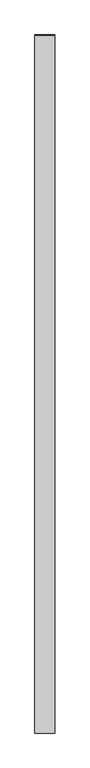
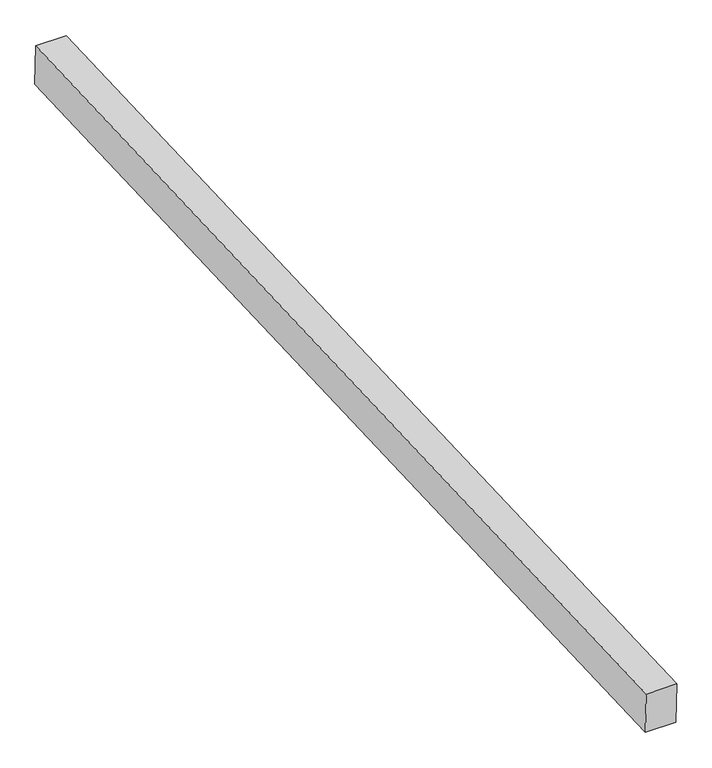
"""IFC4 building model written with IfcOpenShell, lengths in millimetres: proxy geometry, Generic Models 7:Generic Models 1:8:Generic Models 1:8 : Generic Models 7:Generic Models 1:337419:44 : Generic Models 7:Generic Models 1:8:Generic Models 1:8 : Generic Models 7:Generic Models 1:337419:315935."""

import ifcopenshell
import ifcopenshell.guid

model = None  # the IFC model being written
_history = None  # IfcOwnerHistory: only IFC2X3 demands one
_inside = {}  # id of a spatial element -> (the spatial element, [elements in it])
_under = {}  # id of a project, library or spatial element -> (it, [spatial elements below it])
_declared = {}  # id of a project -> (the project, [libraries it declares])
_typed = {}  # id of a type object -> (the type object, [elements of that type])
_made_of = {}  # id of a material, layer set ... -> (it, [elements and type objects made of it])


def new_model(schema):
    """Start an empty IFC model of exactly this schema.

    Asked for "IFC4X3", IfcOpenShell would pick the latest addendum, in which some entities
    have other attributes; the version numbers below select the first issue.
    IFC2X3 requires an IfcOwnerHistory on every rooted entity: one is made here for all.
    """
    global model, _history
    if schema == "IFC4X3":
        model = ifcopenshell.file(schema_version=(4, 3, 0, 0))
    else:
        model = ifcopenshell.file(schema=schema)
    _inside.clear()
    _under.clear()
    _declared.clear()
    _typed.clear()
    _made_of.clear()
    _history = None
    if model.schema == "IFC2X3":
        org = make("IfcOrganization", Name="unknown")
        user = make(
            "IfcPersonAndOrganization",
            ThePerson=make("IfcPerson", FamilyName="unknown"),
            TheOrganization=org,
        )
        app = make(
            "IfcApplication",
            ApplicationDeveloper=org,
            Version="unknown",
            ApplicationFullName="unknown",
            ApplicationIdentifier="unknown",
        )
        _history = make(
            "IfcOwnerHistory",
            OwningUser=user,
            OwningApplication=app,
            ChangeAction="ADDED",
            CreationDate=0,
        )
    return model


def make(cls, **values):
    """One entity of the class cls with the attributes given. An attribute that is None is left unset."""
    return model.create_entity(
        cls, **{name: value for name, value in values.items() if value is not None}
    )


def rooted(cls, **values):
    """An entity with a GlobalId (a new one), such as an element, a storey or a relation."""
    return make(cls, GlobalId=ifcopenshell.guid.new(), OwnerHistory=_history, **values)


def si_unit(unit_type, name, prefix=None):
    """IfcSIUnit, for example si_unit("LENGTHUNIT", "METRE", prefix="MILLI")."""
    return make("IfcSIUnit", UnitType=unit_type, Prefix=prefix, Name=name)


def assignment(units):
    """IfcUnitAssignment: the units of a project."""
    return None if units is None else make("IfcUnitAssignment", Units=units)


def point(xyz):
    """IfcCartesianPoint."""
    return None if xyz is None else make("IfcCartesianPoint", Coordinates=xyz)


def direction(xyz):
    """IfcDirection."""
    return None if xyz is None else make("IfcDirection", DirectionRatios=xyz)


def frame(location, z_axis=None, x_axis=None):
    """IfcAxis2Placement3D, a coordinate frame: its origin and axes. An axis left out is left unset."""
    return make(
        "IfcAxis2Placement3D",
        Location=point(location),
        Axis=direction(z_axis),
        RefDirection=direction(x_axis),
    )


def origin():
    """The frame at (0, 0, 0) with its axes left unset."""
    return frame((0.0, 0.0, 0.0))


def place(relative_to, where):
    """IfcLocalPlacement: puts the frame where relative to a parent placement (None: the world)."""
    return make(
        "IfcLocalPlacement", PlacementRelTo=relative_to, RelativePlacement=where
    )


def context(
    kind, dimensions, precision=None, world=None, true_north=None, identifier=None
):
    """IfcGeometricRepresentationContext, for example the 3D "Model" context."""
    return make(
        "IfcGeometricRepresentationContext",
        ContextIdentifier=identifier,
        ContextType=kind,
        CoordinateSpaceDimension=dimensions,
        Precision=precision,
        WorldCoordinateSystem=world,
        TrueNorth=true_north,
    )


def project(units=None, contexts=None):
    """IfcProject with its units and contexts."""
    return rooted(
        "IfcProject",
        Name="project",
        RepresentationContexts=contexts,
        UnitsInContext=assignment(units),
    )


def spatial(cls, under=None, at=None, **own):
    """A site, building, storey or space (cls), placed at a placement, below another one or the project."""
    s = rooted(cls, ObjectPlacement=at, **own)
    if under is not None:
        _under.setdefault(under.id(), (under, []))[1].append(s)
    return s


def polyline(points):
    """IfcPolyline through the points."""
    return make("IfcPolyline", Points=[point(p) for p in points])


def outline(outer, holes=None, kind="AREA"):
    """IfcArbitraryClosedProfileDef: a profile drawn as a closed curve; with holes, ...WithVoids."""
    if holes is None:
        return make("IfcArbitraryClosedProfileDef", ProfileType=kind, OuterCurve=outer)
    return make(
        "IfcArbitraryProfileDefWithVoids",
        ProfileType=kind,
        OuterCurve=outer,
        InnerCurves=holes,
    )


def extrude(swept, where, along, depth):
    """IfcExtrudedAreaSolid: the profile swept, set in the frame where, extruded along a direction by depth."""
    return make(
        "IfcExtrudedAreaSolid",
        SweptArea=swept,
        Position=where,
        ExtrudedDirection=direction(along),
        Depth=depth,
    )


def shape(context_of_items, identifier, shape_type, items):
    """IfcShapeRepresentation: the items that make up one representation, for example the "Body"."""
    return make(
        "IfcShapeRepresentation",
        ContextOfItems=context_of_items,
        RepresentationIdentifier=identifier,
        RepresentationType=shape_type,
        Items=items,
    )


def source(mapping_origin, context_of_items, identifier, shape_type, items):
    """IfcRepresentationMap: a shape defined once, which mapped items show again and again."""
    return make(
        "IfcRepresentationMap",
        MappingOrigin=mapping_origin,
        MappedRepresentation=shape(context_of_items, identifier, shape_type, items),
    )


def transform(
    local_origin,
    x_axis=None,
    y_axis=None,
    z_axis=None,
    scale=None,
    scale2=None,
    scale3=None,
    uniform=True,
):
    """IfcCartesianTransformationOperator3D, or its non-uniform kind. x_axis, y_axis, z_axis: its Axis1, 2, 3."""
    if uniform:
        return make(
            "IfcCartesianTransformationOperator3D",
            Axis1=direction(x_axis),
            Axis2=direction(y_axis),
            LocalOrigin=point(local_origin),
            Scale=scale,
            Axis3=direction(z_axis),
        )
    return make(
        "IfcCartesianTransformationOperator3DnonUniform",
        Axis1=direction(x_axis),
        Axis2=direction(y_axis),
        LocalOrigin=point(local_origin),
        Scale=scale,
        Axis3=direction(z_axis),
        Scale2=scale2,
        Scale3=scale3,
    )


def mapped(mapping_source, mapping_target):
    """IfcMappedItem: shows the shape of a source again, moved by a transform."""
    return make(
        "IfcMappedItem", MappingSource=mapping_source, MappingTarget=mapping_target
    )


def made_of(thing, what):
    """Note that an element or type object is made of a material, layer set ...; save() writes the relation."""
    if what is not None:
        _made_of.setdefault(what.id(), (what, []))[1].append(thing)
    return thing


def element(
    cls,
    number,
    at=None,
    inside=None,
    cuts=None,
    type_object=None,
    material=None,
    context=None,
    identifier="Body",
    shape_type=None,
    held_by="IfcProductDefinitionShape",
    body=None,
    shapes=None,
    **own,
):
    """One element of the class cls, such as IfcWall. Its Tag is "e" and its number.

    at: its placement. inside: the storey or other place that contains it. cuts: it is an
    opening in that element (IfcRelVoidsElement). A single representation is given by context,
    identifier, shape_type and body (its items); several are given by shapes. held_by: the class
    of the entity that holds the representations. save() writes the other relations.
    """
    e = rooted(cls, Tag="e%d" % number, ObjectPlacement=at, **own)
    if body is not None:
        shapes = [shape(context, identifier, shape_type, body)]
    if shapes is not None:
        e.Representation = make(held_by, Representations=shapes)
    if inside is not None:
        _inside.setdefault(inside.id(), (inside, []))[1].append(e)
    if cuts is not None:
        rooted(
            "IfcRelVoidsElement", RelatingBuildingElement=cuts, RelatedOpeningElement=e
        )
    if type_object is not None:
        _typed.setdefault(type_object.id(), (type_object, []))[1].append(e)
    return made_of(e, material)


def aggregate(whole, parts):
    """IfcRelAggregates: a whole, such as a stair, and the parts it consists of."""
    return rooted("IfcRelAggregates", RelatingObject=whole, RelatedObjects=parts)


def save(model, path):
    """Write the relations noted so far, then the file.

    IfcRelAggregates (storeys below a building ...), IfcRelContainedInSpatialStructure (elements
    in a storey), IfcRelDefinesByType, IfcRelAssociatesMaterial and IfcRelDeclares: one each for
    every whole, place, type object, material and project.
    """
    for whole, parts in _under.values():
        aggregate(whole, parts)
    for where, things in _inside.values():
        rooted(
            "IfcRelContainedInSpatialStructure",
            RelatedElements=things,
            RelatingStructure=where,
        )
    for kind, things in _typed.values():
        rooted("IfcRelDefinesByType", RelatedObjects=things, RelatingType=kind)
    for what, things in _made_of.values():
        rooted("IfcRelAssociatesMaterial", RelatedObjects=things, RelatingMaterial=what)
    for by, libraries in _declared.values():
        rooted("IfcRelDeclares", RelatingContext=by, RelatedDefinitions=libraries)
    model.write(path)


def generic_models_2becdbc0(model_context):
    return source(origin(), model_context, "Body", "SweptSolid", [
        extrude(outline(polyline([(-581229.2495411, 3818.908703), (-576356.3266468, 4021.9471569), (-576348.7597251, 3831.5971524), (-581221.3189223, 3628.5738526), (-581229.2495411, 3818.908703)])), frame((659844.7617239, 0.0, 0.0), z_axis=(1.0, 0.0, 0.0), x_axis=(0.0, 1.0, 0.0)), (0.0, 0.0, 1.0), 139.7),
    ])


if __name__ == "__main__":
    model = new_model("IFC4")
    model_context = context("Model", 3, world=origin())
    ifc_project = project(units=[si_unit("LENGTHUNIT", "METRE", prefix="MILLI")], contexts=[model_context])
    site = spatial("IfcSite", under=ifc_project)
    building = spatial("IfcBuilding", under=site)
    placement = place(None, origin())
    generic_models_shape = generic_models_2becdbc0(model_context)
    element("IfcBuildingElementProxy", 1, Name="Generic Models 7:Generic Models 1:8:Generic Models 1:8 : Generic Models 7:Generic Models 1:337419:44 : Generic Models 7:Generic Models 1:8:Generic Models 1:8 : Generic Models 7:Generic Models 1:337419:315935", ObjectType="Generic Models 7:Generic Models 1:8:Generic Models 1:8 : Generic Models 7:Generic Models 1:337419:44 : Generic Models 7:Generic Models 1:8:Generic Models 1:8 : Generic Models 7:Generic Models 1:337419:315935", at=placement, inside=building, context=model_context, shape_type="MappedRepresentation", body=[
        mapped(generic_models_shape, transform((0.0, 0.0, 0.0), x_axis=(1.0, 0.0, 0.0), y_axis=(0.0, 1.0, 0.0), z_axis=(0.0, 0.0, 1.0))),
    ])
    save(model, "model.ifc")

# Revit data of these elements
# Type "Generic Models 7:Generic Models 1:8:Generic Models 1:8 : Generic Models 7:Generic Models 1:337419:44 : Generic Models 7:Generic Models 1:8:Generic Models 1:8 : Generic Models 7:Generic Models 1:337419:315935"
#   NameOverride = "Generic Models 7:Generic Models 1:8:Generic Models 1:8 : Generic Models 7:Generic Models 1:337419:315935"
#   ObjectTypeOverride = "Generic Models 1:8 : Generic Models 7:Generic Models 1:337419"
#   Reference = "Generic Models 1"
#   Tag = "315935"
# Element 1 (IfcBuildingElementProxy, "Generic Models 7:Generic Models 1:8:Generic Models 1:8 : Generic Models 7:Generic Models 1:337419:44 : Generic Models 7:Generic Models 1:8:Generic Models 1:8 : Generic Models 7:Generic Models 1:337419:315935")
#   Materials on its faces: "5 1/2\" X 7 1/2\" EXTERIOR GRADE GLULAM BEAMS"
# Materials
#   "5 1/2\" X 7 1/2\" EXTERIOR GRADE GLULAM BEAMS": class "Wood", colour RGB 183 134 68, transparency 0, Keynote = "M06181300.01", Description = "Pinus Echinata", Cost = 0
